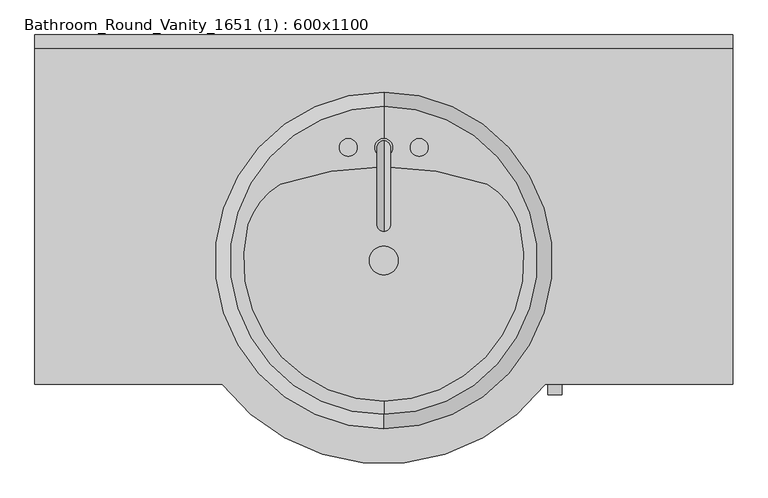
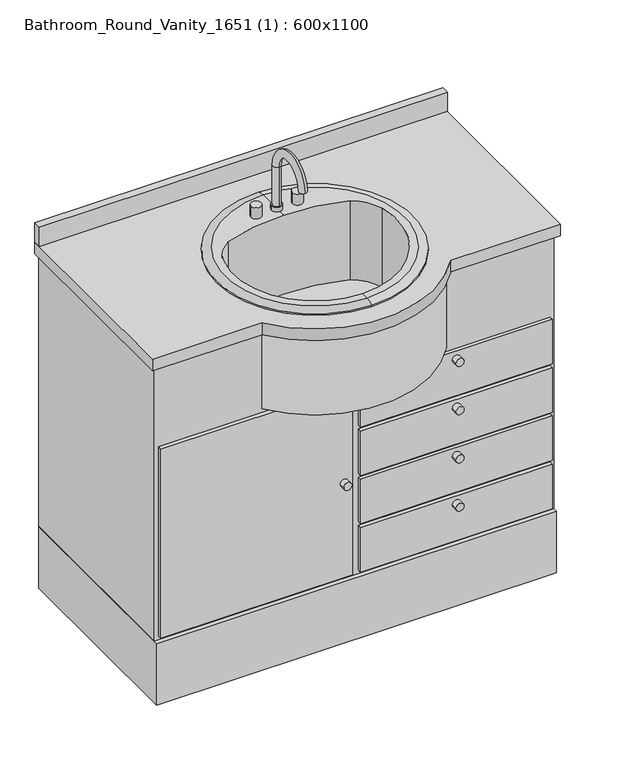
"""IFC4 building model written with IfcOpenShell, lengths in millimetres: furniture geometry, Bathroom_Round_Vanity_1651 (1) : 600x1100."""

import ifcopenshell
import ifcopenshell.guid

model = None  # the IFC model being written
_history = None  # IfcOwnerHistory: only IFC2X3 demands one
_inside = {}  # id of a spatial element -> (the spatial element, [elements in it])
_under = {}  # id of a project, library or spatial element -> (it, [spatial elements below it])
_declared = {}  # id of a project -> (the project, [libraries it declares])
_typed = {}  # id of a type object -> (the type object, [elements of that type])
_made_of = {}  # id of a material, layer set ... -> (it, [elements and type objects made of it])


def new_model(schema):
    """Start an empty IFC model of exactly this schema.

    Asked for "IFC4X3", IfcOpenShell would pick the latest addendum, in which some entities
    have other attributes; the version numbers below select the first issue.
    IFC2X3 requires an IfcOwnerHistory on every rooted entity: one is made here for all.
    """
    global model, _history
    if schema == "IFC4X3":
        model = ifcopenshell.file(schema_version=(4, 3, 0, 0))
    else:
        model = ifcopenshell.file(schema=schema)
    _inside.clear()
    _under.clear()
    _declared.clear()
    _typed.clear()
    _made_of.clear()
    _history = None
    if model.schema == "IFC2X3":
        org = make("IfcOrganization", Name="unknown")
        user = make(
            "IfcPersonAndOrganization",
            ThePerson=make("IfcPerson", FamilyName="unknown"),
            TheOrganization=org,
        )
        app = make(
            "IfcApplication",
            ApplicationDeveloper=org,
            Version="unknown",
            ApplicationFullName="unknown",
            ApplicationIdentifier="unknown",
        )
        _history = make(
            "IfcOwnerHistory",
            OwningUser=user,
            OwningApplication=app,
            ChangeAction="ADDED",
            CreationDate=0,
        )
    return model


def make(cls, **values):
    """One entity of the class cls with the attributes given. An attribute that is None is left unset."""
    return model.create_entity(
        cls, **{name: value for name, value in values.items() if value is not None}
    )


def rooted(cls, **values):
    """An entity with a GlobalId (a new one), such as an element, a storey or a relation."""
    return make(cls, GlobalId=ifcopenshell.guid.new(), OwnerHistory=_history, **values)


def si_unit(unit_type, name, prefix=None):
    """IfcSIUnit, for example si_unit("LENGTHUNIT", "METRE", prefix="MILLI")."""
    return make("IfcSIUnit", UnitType=unit_type, Prefix=prefix, Name=name)


def assignment(units):
    """IfcUnitAssignment: the units of a project."""
    return None if units is None else make("IfcUnitAssignment", Units=units)


def point(xyz):
    """IfcCartesianPoint."""
    return None if xyz is None else make("IfcCartesianPoint", Coordinates=xyz)


def direction(xyz):
    """IfcDirection."""
    return None if xyz is None else make("IfcDirection", DirectionRatios=xyz)


def frame(location, z_axis=None, x_axis=None):
    """IfcAxis2Placement3D, a coordinate frame: its origin and axes. An axis left out is left unset."""
    return make(
        "IfcAxis2Placement3D",
        Location=point(location),
        Axis=direction(z_axis),
        RefDirection=direction(x_axis),
    )


def frame_2d(location, x_axis=None):
    """IfcAxis2Placement2D, a coordinate frame in the plane: its origin and x axis."""
    return make(
        "IfcAxis2Placement2D", Location=point(location), RefDirection=direction(x_axis)
    )


def origin():
    """The frame at (0, 0, 0) with its axes left unset."""
    return frame((0.0, 0.0, 0.0))


def origin_with_axes():
    """The frame at (0, 0, 0) with the z axis (0, 0, 1) and the x axis (1, 0, 0) written out."""
    return frame((0.0, 0.0, 0.0), z_axis=(0.0, 0.0, 1.0), x_axis=(1.0, 0.0, 0.0))


def place(relative_to, where):
    """IfcLocalPlacement: puts the frame where relative to a parent placement (None: the world)."""
    return make(
        "IfcLocalPlacement", PlacementRelTo=relative_to, RelativePlacement=where
    )


def context(
    kind, dimensions, precision=None, world=None, true_north=None, identifier=None
):
    """IfcGeometricRepresentationContext, for example the 3D "Model" context."""
    return make(
        "IfcGeometricRepresentationContext",
        ContextIdentifier=identifier,
        ContextType=kind,
        CoordinateSpaceDimension=dimensions,
        Precision=precision,
        WorldCoordinateSystem=world,
        TrueNorth=true_north,
    )


def project(units=None, contexts=None):
    """IfcProject with its units and contexts."""
    return rooted(
        "IfcProject",
        Name="project",
        RepresentationContexts=contexts,
        UnitsInContext=assignment(units),
    )


def spatial(cls, under=None, at=None, **own):
    """A site, building, storey or space (cls), placed at a placement, below another one or the project."""
    s = rooted(cls, ObjectPlacement=at, **own)
    if under is not None:
        _under.setdefault(under.id(), (under, []))[1].append(s)
    return s


def polyline(points):
    """IfcPolyline through the points."""
    return make("IfcPolyline", Points=[point(p) for p in points])


def circle_curve(where, radius):
    """IfcCircle in the frame where."""
    return make("IfcCircle", Position=where, Radius=radius)


def ellipse_curve(where, semi_axis1, semi_axis2):
    """IfcEllipse in the frame where."""
    return make(
        "IfcEllipse", Position=where, SemiAxis1=semi_axis1, SemiAxis2=semi_axis2
    )


def trimmed(basis, trim1, trim2, sense, master):
    """IfcTrimmedCurve: the piece of a basis curve between two trims."""
    return make(
        "IfcTrimmedCurve",
        BasisCurve=basis,
        Trim1=trim1,
        Trim2=trim2,
        SenseAgreement=sense,
        MasterRepresentation=master,
    )


def segment(curve, same_sense, transition):
    """IfcCompositeCurveSegment."""
    return make(
        "IfcCompositeCurveSegment",
        Transition=transition,
        SameSense=same_sense,
        ParentCurve=curve,
    )


def composite_curve(segments, self_intersect=None):
    """IfcCompositeCurve: segments joined end to end."""
    return make("IfcCompositeCurve", Segments=segments, SelfIntersect=self_intersect)


def outline(outer, holes=None, kind="AREA"):
    """IfcArbitraryClosedProfileDef: a profile drawn as a closed curve; with holes, ...WithVoids."""
    if holes is None:
        return make("IfcArbitraryClosedProfileDef", ProfileType=kind, OuterCurve=outer)
    return make(
        "IfcArbitraryProfileDefWithVoids",
        ProfileType=kind,
        OuterCurve=outer,
        InnerCurves=holes,
    )


def extrude(swept, where, along, depth):
    """IfcExtrudedAreaSolid: the profile swept, set in the frame where, extruded along a direction by depth."""
    return make(
        "IfcExtrudedAreaSolid",
        SweptArea=swept,
        Position=where,
        ExtrudedDirection=direction(along),
        Depth=depth,
    )


def shape(context_of_items, identifier, shape_type, items):
    """IfcShapeRepresentation: the items that make up one representation, for example the "Body"."""
    return make(
        "IfcShapeRepresentation",
        ContextOfItems=context_of_items,
        RepresentationIdentifier=identifier,
        RepresentationType=shape_type,
        Items=items,
    )


def source(mapping_origin, context_of_items, identifier, shape_type, items):
    """IfcRepresentationMap: a shape defined once, which mapped items show again and again."""
    return make(
        "IfcRepresentationMap",
        MappingOrigin=mapping_origin,
        MappedRepresentation=shape(context_of_items, identifier, shape_type, items),
    )


def transform(
    local_origin,
    x_axis=None,
    y_axis=None,
    z_axis=None,
    scale=None,
    scale2=None,
    scale3=None,
    uniform=True,
):
    """IfcCartesianTransformationOperator3D, or its non-uniform kind. x_axis, y_axis, z_axis: its Axis1, 2, 3."""
    if uniform:
        return make(
            "IfcCartesianTransformationOperator3D",
            Axis1=direction(x_axis),
            Axis2=direction(y_axis),
            LocalOrigin=point(local_origin),
            Scale=scale,
            Axis3=direction(z_axis),
        )
    return make(
        "IfcCartesianTransformationOperator3DnonUniform",
        Axis1=direction(x_axis),
        Axis2=direction(y_axis),
        LocalOrigin=point(local_origin),
        Scale=scale,
        Axis3=direction(z_axis),
        Scale2=scale2,
        Scale3=scale3,
    )


def mapped(mapping_source, mapping_target):
    """IfcMappedItem: shows the shape of a source again, moved by a transform."""
    return make(
        "IfcMappedItem", MappingSource=mapping_source, MappingTarget=mapping_target
    )


def made_of(thing, what):
    """Note that an element or type object is made of a material, layer set ...; save() writes the relation."""
    if what is not None:
        _made_of.setdefault(what.id(), (what, []))[1].append(thing)
    return thing


def element(
    cls,
    number,
    at=None,
    inside=None,
    cuts=None,
    type_object=None,
    material=None,
    context=None,
    identifier="Body",
    shape_type=None,
    held_by="IfcProductDefinitionShape",
    body=None,
    shapes=None,
    **own,
):
    """One element of the class cls, such as IfcWall. Its Tag is "e" and its number.

    at: its placement. inside: the storey or other place that contains it. cuts: it is an
    opening in that element (IfcRelVoidsElement). A single representation is given by context,
    identifier, shape_type and body (its items); several are given by shapes. held_by: the class
    of the entity that holds the representations. save() writes the other relations.
    """
    e = rooted(cls, Tag="e%d" % number, ObjectPlacement=at, **own)
    if body is not None:
        shapes = [shape(context, identifier, shape_type, body)]
    if shapes is not None:
        e.Representation = make(held_by, Representations=shapes)
    if inside is not None:
        _inside.setdefault(inside.id(), (inside, []))[1].append(e)
    if cuts is not None:
        rooted(
            "IfcRelVoidsElement", RelatingBuildingElement=cuts, RelatedOpeningElement=e
        )
    if type_object is not None:
        _typed.setdefault(type_object.id(), (type_object, []))[1].append(e)
    return made_of(e, material)


def aggregate(whole, parts):
    """IfcRelAggregates: a whole, such as a stair, and the parts it consists of."""
    return rooted("IfcRelAggregates", RelatingObject=whole, RelatedObjects=parts)


def save(model, path):
    """Write the relations noted so far, then the file.

    IfcRelAggregates (storeys below a building ...), IfcRelContainedInSpatialStructure (elements
    in a storey), IfcRelDefinesByType, IfcRelAssociatesMaterial and IfcRelDeclares: one each for
    every whole, place, type object, material and project.
    """
    for whole, parts in _under.values():
        aggregate(whole, parts)
    for where, things in _inside.values():
        rooted(
            "IfcRelContainedInSpatialStructure",
            RelatedElements=things,
            RelatingStructure=where,
        )
    for kind, things in _typed.values():
        rooted("IfcRelDefinesByType", RelatedObjects=things, RelatingType=kind)
    for what, things in _made_of.values():
        rooted("IfcRelAssociatesMaterial", RelatedObjects=things, RelatingMaterial=what)
    for by, libraries in _declared.values():
        rooted("IfcRelDeclares", RelatingContext=by, RelatedDefinitions=libraries)
    model.write(path)


def plane_surface(at):
    """IfcPlane: the flat surface through the origin of the frame at, square to its z axis."""
    return make("IfcPlane", Position=at)


def cylinder_surface(at, radius):
    """IfcCylindricalSurface: all points at the distance radius from the z axis of the frame at."""
    return make("IfcCylindricalSurface", Position=at, Radius=radius)


def revolved_surface(curve, axis_point, axis_direction):
    """IfcSurfaceOfRevolution: the curve turned about the line through axis_point along axis_direction."""
    return make(
        "IfcSurfaceOfRevolution",
        SweptCurve=make("IfcArbitraryOpenProfileDef", ProfileType="CURVE", Curve=curve),
        AxisPosition=make("IfcAxis1Placement", Location=point(axis_point), Axis=direction(axis_direction)),
    )


def advanced_brep(points, edges, surfaces, faces):
    """IfcAdvancedBrep: a solid bounded by faces that lie on surfaces and meet in shared edges.

    An edge is (start, end): straight between two places in points (the first is 0);
    or (start, end, curve); or (start, end, curve, False) where it runs against its curve.
    A face is (place in surfaces, loops), or (place, loops, False) where it looks against
    its surface's normal. A loop lists edges by number (the first is 1), with a minus sign
    where the edge is run from its end to its start. The first loop is the outer one.
    """
    corners = [point(p) for p in points]
    vertices = [make("IfcVertexPoint", VertexGeometry=c) for c in corners]
    made = []
    for start, end, *more in edges:
        made.append(
            make(
                "IfcEdgeCurve",
                EdgeStart=vertices[start],
                EdgeEnd=vertices[end],
                EdgeGeometry=more[0] if more else make("IfcPolyline", Points=[corners[start], corners[end]]),
                SameSense=more[1] if len(more) > 1 else True,
            )
        )
    hull = []
    for where, loops, *sense in faces:
        bounds = []
        for j, loop in enumerate(loops):
            ring = [make("IfcOrientedEdge", EdgeElement=made[abs(k) - 1], Orientation=k > 0) for k in loop]
            bounds.append(
                make(
                    "IfcFaceOuterBound" if j == 0 else "IfcFaceBound",
                    Bound=make("IfcEdgeLoop", EdgeList=ring),
                    Orientation=True,
                )
            )
        hull.append(make("IfcAdvancedFace", Bounds=bounds, FaceSurface=surfaces[where], SameSense=sense[0] if sense else True))
    return make("IfcAdvancedBrep", Outer=make("IfcClosedShell", CfsFaces=hull))


def bathroom_round_vanity_1651_1_600x1100_b041f343(model_context):
    return source(origin(), model_context, "Body", "SolidModel", [
        advanced_brep(
        [(94.9377049, -170.6504315, 909.525), (94.9377049, -151.6004315, 909.525), (94.9377049, -170.6504315, 1022.2375), (94.9377049, -151.6004315, 1022.2375), (94.9377049, -262.4406462, 1022.2375), (94.9377049, -281.4906462, 1022.2375)],
        [
            (0, 1, circle_curve(frame((94.9377049, -161.1254315, 909.525), z_axis=(0.0, 0.0, -1.0), x_axis=(0.0, 1.0, 0.0)), 9.525)),
            (1, 0, circle_curve(frame((94.9377049, -161.1254315, 909.525), z_axis=(0.0, 0.0, -1.0), x_axis=(0.0, 1.0, 0.0)), 9.525)),
            (0, 2),
            (2, 3, circle_curve(frame((94.9377049, -161.1254315, 1022.2375), z_axis=(0.0, 0.0, -1.0), x_axis=(0.0, 1.0, 0.0)), 9.525)),
            (3, 1),
            (3, 2, circle_curve(frame((94.9377049, -161.1254315, 1022.2375), z_axis=(0.0, 0.0, -1.0), x_axis=(0.0, 1.0, 0.0)), 9.525)),
            (4, 5, circle_curve(frame((94.9377049, -271.9656462, 1022.2375), z_axis=(0.0, 0.0, -1.0), x_axis=(0.0, -1.0, 0.0)), 9.525)),
            (5, 4, circle_curve(frame((94.9377049, -271.9656462, 1022.2375), z_axis=(0.0, 0.0, -1.0), x_axis=(0.0, -1.0, 0.0)), 9.525)),
            (5, 3, circle_curve(frame((94.9377049, -216.5455388, 1022.2375), z_axis=(-1.0, 0.0, 0.0), x_axis=(0.0, 1.0, 0.0)), 64.9451073)),
            (2, 4, circle_curve(frame((94.9377049, -216.5455388, 1022.2375), z_axis=(1.0, 0.0, 0.0), x_axis=(0.0, 1.0, 0.0)), 45.8951073)),
        ],
        [
            plane_surface(frame((94.9377049, -170.6504315, 909.525), z_axis=(0.0, 0.0, -1.0), x_axis=(1.0, 0.0, 0.0))),
            cylinder_surface(frame((94.9377049, -161.1254315, 909.525), z_axis=(0.0, 0.0, -1.0), x_axis=(0.0, 1.0, 0.0)), 9.525),
            plane_surface(frame((94.9377049, -216.5455388, 1022.2375), z_axis=(0.0, 0.0, -1.0), x_axis=(0.0, -1.0, 0.0))),
            revolved_surface(trimmed(ellipse_curve(frame((94.9377049, -161.1254315, 1022.2375), z_axis=(0.0, 0.0, -1.0), x_axis=(0.0, 1.0, 0.0)), 9.525, 9.525), [point((94.9377049, -170.6504315, 1022.2375))], [point((94.9377049, -151.6004315, 1022.2375))], True, "CARTESIAN"), (94.9377049, -216.5455388, 1022.2375), (1.0, 0.0, 0.0)),
            revolved_surface(trimmed(ellipse_curve(frame((94.9377049, -161.1254315, 1022.2375), z_axis=(0.0, 0.0, -1.0), x_axis=(0.0, 1.0, 0.0)), 9.525, 9.525), [point((94.9377049, -151.6004315, 1022.2375))], [point((94.9377049, -170.6504315, 1022.2375))], True, "CARTESIAN"), (94.9377049, -216.5455388, 1022.2375), (1.0, 0.0, 0.0)),
        ],
        [
            (0, [[1, 2]]),
            (1, [[-1, 3, 4, 5]]),
            (1, [[-2, -5, 6, -3]]),
            (2, [[7, 8]]),
            (3, [[9, -4, 10, -8]]),
            (4, [[-10, -6, -9, -7]]),
        ],
    ),
        extrude(outline(composite_curve([segment(trimmed(circle_curve(frame_2d((94.9377049, -161.1254315)), 12.7), [point((82.2377049, -161.1254315))], [point((107.6377049, -161.1254315))], False, "CARTESIAN"), True, "CONTINUOUS"), segment(trimmed(circle_curve(frame_2d((94.9377049, -161.1254315)), 12.7), [point((107.6377049, -161.1254315))], [point((82.2377049, -161.1254315))], False, "CARTESIAN"), True, "CONTINUOUS")], self_intersect=False)), frame((0.0, 0.0, 909.525), z_axis=(0.0, 0.0, 1.0), x_axis=(1.0, 0.0, 0.0)), (0.0, 0.0, 1.0), 12.2352909),
        extrude(outline(composite_curve([segment(trimmed(circle_curve(frame_2d((44.1377049, -161.1254315)), 12.7), [point((31.4377049, -161.1254315))], [point((56.8377049, -161.1254315))], False, "CARTESIAN"), True, "CONTINUOUS"), segment(trimmed(circle_curve(frame_2d((44.1377049, -161.1254315)), 12.7), [point((56.8377049, -161.1254315))], [point((31.4377049, -161.1254315))], False, "CARTESIAN"), True, "CONTINUOUS")], self_intersect=False)), frame((0.0, 0.0, 909.525), z_axis=(0.0, 0.0, 1.0), x_axis=(1.0, 0.0, 0.0)), (0.0, 0.0, 1.0), 28.575),
        extrude(outline(composite_curve([segment(trimmed(circle_curve(frame_2d((145.7377049, -161.1254315)), 12.7), [point((133.0377049, -161.1254315))], [point((158.4377049, -161.1254315))], False, "CARTESIAN"), True, "CONTINUOUS"), segment(trimmed(circle_curve(frame_2d((145.7377049, -161.1254315)), 12.7), [point((158.4377049, -161.1254315))], [point((133.0377049, -161.1254315))], False, "CARTESIAN"), True, "CONTINUOUS")], self_intersect=False)), frame((0.0, 0.0, 909.525), z_axis=(0.0, 0.0, 1.0), x_axis=(1.0, 0.0, 0.0)), (0.0, 0.0, 1.0), 28.575),
        extrude(outline(composite_curve([segment(trimmed(circle_curve(frame_2d((94.9377049, -323.0504315)), 20.6375), [point((74.3002049, -323.0504315))], [point((115.5752049, -323.0504315))], False, "CARTESIAN"), True, "CONTINUOUS"), segment(trimmed(circle_curve(frame_2d((94.9377049, -323.0504315)), 20.6375), [point((115.5752049, -323.0504315))], [point((74.3002049, -323.0504315))], False, "CARTESIAN"), True, "CONTINUOUS")], self_intersect=False)), frame((0.0, 0.0, 684.1), z_axis=(0.0, 0.0, 1.0), x_axis=(1.0, 0.0, 0.0)), (0.0, 0.0, 1.0), 21.1842611),
        advanced_brep(
        [(94.9377049, -543.6051593, 909.525), (94.9377049, -102.4957037, 909.525), (94.9377049, -81.7504315, 903.96875), (94.9377049, -564.3504315, 903.96875), (94.9377049, -524.4587205, 909.525), (-99.884377, -271.9656462, 909.525), (-53.8675289, -214.1320102, 909.525), (94.9377049, -188.9519451, 909.525), (243.7429387, -214.1320102, 909.525), (289.7597868, -271.9656462, 909.525), (94.9377049, -515.3445528, 684.1), (94.9377049, -130.7563102, 684.1), (94.9377049, -323.0504315, 684.1), (94.9377049, -535.9008861, 705.2842611), (94.9377049, -110.1999769, 705.2842611), (94.9377049, -552.4441815, 900.0), (94.9377049, -93.6566815, 900.0), (94.9377049, -564.3504315, 900.0), (94.9377049, -81.7504315, 900.0), (243.7429387, -214.1320102, 705.2842611), (-53.8675289, -214.1320102, 705.2842611), (-99.884377, -271.9656462, 705.2842611), (289.7597868, -271.9656462, 705.2842611)],
        [
            (0, 1, circle_curve(frame((94.9377049, -323.0504315, 909.525), z_axis=(0.0, 0.0, -1.0), x_axis=(0.0, 1.0, 0.0)), 220.5547278)),
            (1, 2, circle_curve(frame((94.9377049, -98.7806884, 881.889434), z_axis=(-1.0, 0.0, 0.0), x_axis=(0.0, 1.0, 0.0)), 27.8841505)),
            (2, 3, circle_curve(frame((94.9377049, -323.0504315, 903.96875), z_axis=(0.0, 0.0, 1.0), x_axis=(0.0, 1.0, 0.0)), 241.3)),
            (3, 0, circle_curve(frame((94.9377049, -547.3201745, 881.889434), z_axis=(-1.0, 0.0, 0.0), x_axis=(0.0, -1.0, 0.0)), 27.8841505)),
            (1, 0, circle_curve(frame((94.9377049, -323.0504315, 909.525), z_axis=(0.0, 0.0, -1.0), x_axis=(0.0, 1.0, 0.0)), 220.5547278)),
            (3, 2, circle_curve(frame((94.9377049, -323.0504315, 903.96875), z_axis=(0.0, 0.0, 1.0), x_axis=(0.0, 1.0, 0.0)), 241.3)),
            (0, 4),
            (4, 5, circle_curve(frame((94.9377049, -323.0504315, 909.525), z_axis=(0.0, 0.0, -1.0), x_axis=(1.0, 0.0, 0.0)), 201.408289)),
            (5, 6, circle_curve(frame((-0.3450667, -303.9426335, 909.525), z_axis=(0.0, 0.0, -1.0), x_axis=(1.0, 0.0, 0.0)), 104.5495194)),
            (6, 7, circle_curve(frame((94.9377049, -641.2349961, 909.525), z_axis=(0.0, 0.0, -1.0), x_axis=(1.0, 0.0, 0.0)), 452.283051)),
            (7, 1),
            (7, 8, circle_curve(frame((94.9377049, -641.2349961, 909.525), z_axis=(0.0, 0.0, -1.0), x_axis=(1.0, 0.0, 0.0)), 452.283051)),
            (8, 9, circle_curve(frame((190.2204765, -303.9426335, 909.525), z_axis=(0.0, 0.0, -1.0), x_axis=(1.0, 0.0, 0.0)), 104.5495194)),
            (9, 4, circle_curve(frame((94.9377049, -323.0504315, 909.525), z_axis=(0.0, 0.0, -1.0), x_axis=(1.0, 0.0, 0.0)), 201.408289)),
            (10, 11, circle_curve(frame((94.9377049, -323.0504315, 684.1), z_axis=(0.0, 0.0, -1.0), x_axis=(0.0, 1.0, 0.0)), 192.2941213)),
            (11, 12),
            (12, 10),
            (11, 10, circle_curve(frame((94.9377049, -323.0504315, 684.1), z_axis=(0.0, 0.0, -1.0), x_axis=(0.0, 1.0, 0.0)), 192.2941213)),
            (10, 13, circle_curve(frame((94.9377049, -515.3445528, 704.6656396), z_axis=(-1.0, 0.0, 0.0), x_axis=(0.0, -1.0, 0.0)), 20.5656396)),
            (13, 14, circle_curve(frame((94.9377049, -323.0504315, 705.2842611), z_axis=(0.0, 0.0, -1.0), x_axis=(0.0, 1.0, 0.0)), 212.8504546)),
            (14, 11, circle_curve(frame((94.9377049, -130.7563102, 704.6656396), z_axis=(-1.0, 0.0, 0.0), x_axis=(0.0, 1.0, 0.0)), 20.5656396)),
            (14, 13, circle_curve(frame((94.9377049, -323.0504315, 705.2842611), z_axis=(0.0, 0.0, -1.0), x_axis=(0.0, 1.0, 0.0)), 212.8504546)),
            (13, 15),
            (15, 16, circle_curve(frame((94.9377049, -323.0504315, 900.0), z_axis=(0.0, 0.0, -1.0), x_axis=(0.0, 1.0, 0.0)), 229.39375)),
            (16, 14),
            (16, 15, circle_curve(frame((94.9377049, -323.0504315, 900.0), z_axis=(0.0, 0.0, -1.0), x_axis=(0.0, 1.0, 0.0)), 229.39375)),
            (15, 17),
            (17, 18, circle_curve(frame((94.9377049, -323.0504315, 900.0), z_axis=(0.0, 0.0, -1.0), x_axis=(0.0, 1.0, 0.0)), 241.3)),
            (18, 16),
            (18, 17, circle_curve(frame((94.9377049, -323.0504315, 900.0), z_axis=(0.0, 0.0, -1.0), x_axis=(0.0, 1.0, 0.0)), 241.3)),
            (2, 18),
            (17, 3),
            (19, 20, circle_curve(frame((94.9377049, -641.2349961, 705.2842611), z_axis=(0.0, 0.0, 1.0), x_axis=(1.0, 0.0, 0.0)), 452.283051)),
            (20, 21, circle_curve(frame((-0.3450667, -303.9426335, 705.2842611), z_axis=(0.0, 0.0, 1.0), x_axis=(1.0, 0.0, 0.0)), 104.5495194)),
            (21, 22, circle_curve(frame((94.9377049, -323.0504315, 705.2842611), z_axis=(0.0, 0.0, 1.0), x_axis=(1.0, 0.0, 0.0)), 201.408289)),
            (22, 19, circle_curve(frame((190.2204765, -303.9426335, 705.2842611), z_axis=(0.0, 0.0, 1.0), x_axis=(1.0, 0.0, 0.0)), 104.5495194)),
            (19, 8),
            (6, 20),
            (5, 21),
            (9, 22),
        ],
        [
            revolved_surface(trimmed(ellipse_curve(frame((94.9377049, -98.7806884, 881.889434), z_axis=(1.0, 0.0, 0.0), x_axis=(0.0, 1.0, 0.0)), 27.8841505, 27.8841505), [point((94.9377049, -81.7504315, 903.96875))], [point((94.9377049, -102.4957037, 909.525))], True, "CARTESIAN"), (94.9377049, -323.0504315, 909.525), (0.0, 0.0, 1.0)),
            plane_surface(frame((94.9377049, -323.0504315, 909.525), z_axis=(0.0, 0.0, 1.0), x_axis=(0.0, 1.0, 0.0))),
            plane_surface(frame((94.9377049, -323.0504315, 684.1), z_axis=(0.0, 0.0, -1.0), x_axis=(0.0, 1.0, 0.0))),
            revolved_surface(trimmed(ellipse_curve(frame((94.9377049, -130.7563102, 704.6656396), z_axis=(1.0, 0.0, 0.0), x_axis=(0.0, 1.0, 0.0)), 20.5656396, 20.5656396), [point((94.9377049, -130.7563102, 684.1))], [point((94.9377049, -110.1999769, 705.2842611))], True, "CARTESIAN"), (94.9377049, -323.0504315, 909.525), (0.0, 0.0, 1.0)),
            revolved_surface(polyline([(94.9377049, -110.1999769, 705.2842611), (94.9377049, -93.6566815, 900.0)]), (94.9377049, -323.0504315, 909.525), (0.0, 0.0, 1.0)),
            plane_surface(frame((94.9377049, -323.0504315, 900.0), z_axis=(0.0, 0.0, -1.0), x_axis=(0.0, 1.0, 0.0))),
            cylinder_surface(frame((94.9377049, -323.0504315, 909.525), z_axis=(0.0, 0.0, 1.0), x_axis=(0.0, 1.0, 0.0)), 241.3),
            plane_surface(frame((547.2207559, -641.2349961, 705.2842611), z_axis=(0.0, 0.0, 1.0), x_axis=(0.0, -1.0, 0.0))),
            revolved_surface(polyline([(547.2207559, -641.2349961, 909.525), (547.2207559, -641.2349961, 705.2842611)]), (94.9377049, -641.2349961, 705.2842611), (0.0, 0.0, 1.0)),
            revolved_surface(polyline([(104.20445269999999, -303.9426335, 909.525), (104.20445269999999, -303.9426335, 705.2842611)]), (-0.3450667, -303.9426335, 705.2842611), (0.0, 0.0, 1.0)),
            revolved_surface(polyline([(296.3459939, -323.0504315, 909.525), (296.3459939, -323.0504315, 705.2842611)]), (94.9377049, -323.0504315, 705.2842611), (0.0, 0.0, 1.0)),
            revolved_surface(polyline([(294.76999589999997, -303.9426335, 909.525), (294.76999589999997, -303.9426335, 705.2842611)]), (190.2204765, -303.9426335, 705.2842611), (0.0, 0.0, 1.0)),
        ],
        [
            (0, [[1, 2, 3, 4]]),
            (0, [[-2, 5, -4, 6]]),
            (1, [[-1, 7, 8, 9, 10, 11]]),
            (1, [[-5, -11, 12, 13, 14, -7]]),
            (2, [[15, 16, 17]]),
            (2, [[-16, 18, -17]]),
            (3, [[-15, 19, 20, 21]]),
            (3, [[-18, -21, 22, -19]]),
            (4, [[-20, 23, 24, 25]]),
            (4, [[-22, -25, 26, -23]]),
            (5, [[-24, 27, 28, 29]]),
            (5, [[-26, -29, 30, -27]]),
            (6, [[-3, 31, -28, 32]]),
            (6, [[-6, -32, -30, -31]]),
            (7, [[33, 34, 35, 36]]),
            (8, [[-33, 37, -12, -10, 38]]),
            (9, [[-34, -38, -9, 39]]),
            (10, [[-35, -39, -8, -14, 40]]),
            (11, [[-36, -40, -13, -37]]),
        ],
    ),
        extrude(outline(composite_curve([segment(trimmed(circle_curve(frame_2d((640.0, 339.9377049)), 10.0), [point((640.0, 329.9377049))], [point((640.0, 349.9377049))], False, "CARTESIAN"), True, "CONTINUOUS"), segment(trimmed(circle_curve(frame_2d((640.0, 339.9377049)), 10.0), [point((640.0, 349.9377049))], [point((640.0, 329.9377049))], False, "CARTESIAN"), True, "CONTINUOUS")], self_intersect=False)), frame((0.0, -515.0, 0.0), z_axis=(0.0, 1.0, 0.0), x_axis=(0.0, 0.0, 1.0)), (0.0, 0.0, 1.0), 15.0),
        extrude(outline(composite_curve([segment(trimmed(circle_curve(frame_2d((515.0, 339.9377049)), 10.0), [point((515.0, 329.9377049))], [point((515.0, 349.9377049))], False, "CARTESIAN"), True, "CONTINUOUS"), segment(trimmed(circle_curve(frame_2d((515.0, 339.9377049)), 10.0), [point((515.0, 349.9377049))], [point((515.0, 329.9377049))], False, "CARTESIAN"), True, "CONTINUOUS")], self_intersect=False)), frame((0.0, -515.0, 0.0), z_axis=(0.0, 1.0, 0.0), x_axis=(0.0, 0.0, 1.0)), (0.0, 0.0, 1.0), 15.0),
        extrude(outline(composite_curve([segment(trimmed(circle_curve(frame_2d((390.0, 339.9377049)), 10.0), [point((390.0, 329.9377049))], [point((390.0, 349.9377049))], False, "CARTESIAN"), True, "CONTINUOUS"), segment(trimmed(circle_curve(frame_2d((390.0, 339.9377049)), 10.0), [point((390.0, 349.9377049))], [point((390.0, 329.9377049))], False, "CARTESIAN"), True, "CONTINUOUS")], self_intersect=False)), frame((0.0, -515.0, 0.0), z_axis=(0.0, 1.0, 0.0), x_axis=(0.0, 0.0, 1.0)), (0.0, 0.0, 1.0), 15.0),
        extrude(outline(composite_curve([segment(polyline([(594.9377049, 0.0), (594.9377049, -500.0), (326.334637, -500.0)]), True, "CONTINUOUS"), segment(trimmed(circle_curve(frame_2d((94.9377049, -323.0504315)), 291.3), [point((326.334637, -500.0))], [point((-136.4592272, -500.0))], False, "CARTESIAN"), True, "CONTINUOUS"), segment(polyline([(-136.4592272, -500.0), (-405.0622951, -500.0), (-405.0622951, 0.0), (594.9377049, 0.0)]), True, "CONTINUOUS")], self_intersect=False), holes=[composite_curve([segment(trimmed(circle_curve(frame_2d((94.9377049, -323.0504315)), 220.5547278), [point((94.9377049, -102.4957037))], [point((94.9377049, -543.6051593))], True, "CARTESIAN"), True, "CONTINUOUS"), segment(trimmed(circle_curve(frame_2d((94.9377049, -323.0504315)), 220.5547278), [point((94.9377049, -543.6051593))], [point((94.9377049, -102.4957037))], True, "CARTESIAN"), True, "CONTINUOUS")], self_intersect=False)]), frame((0.0, 0.0, 870.0), z_axis=(0.0, 0.0, 1.0), x_axis=(1.0, 0.0, 0.0)), (0.0, 0.0, 1.0), 30.0),
        extrude(outline(composite_curve([segment(trimmed(circle_curve(frame_2d((265.0, 339.9377049)), 10.0), [point((265.0, 329.9377049))], [point((265.0, 349.9377049))], False, "CARTESIAN"), True, "CONTINUOUS"), segment(trimmed(circle_curve(frame_2d((265.0, 339.9377049)), 10.0), [point((265.0, 349.9377049))], [point((265.0, 329.9377049))], False, "CARTESIAN"), True, "CONTINUOUS")], self_intersect=False)), frame((0.0, -515.0, 0.0), z_axis=(0.0, 1.0, 0.0), x_axis=(0.0, 0.0, 1.0)), (0.0, 0.0, 1.0), 15.0),
        extrude(outline(composite_curve([segment(trimmed(circle_curve(frame_2d((415.0, 64.9377049)), 10.0), [point((415.0, 74.9377049))], [point((415.0, 54.9377049))], False, "CARTESIAN"), True, "CONTINUOUS"), segment(trimmed(circle_curve(frame_2d((415.0, 64.9377049)), 10.0), [point((415.0, 54.9377049))], [point((415.0, 74.9377049))], False, "CARTESIAN"), True, "CONTINUOUS")], self_intersect=False)), frame((0.0, -515.0, 0.0), z_axis=(0.0, 1.0, 0.0), x_axis=(0.0, 0.0, 1.0)), (0.0, 0.0, 1.0), 15.0),
        extrude(outline(polyline([(574.9377049, -500.0), (104.9377049, -500.0), (104.9377049, -490.0), (574.9377049, -490.0), (574.9377049, -500.0)])), frame((0.0, 0.0, 170.0), z_axis=(0.0, 0.0, 1.0), x_axis=(1.0, 0.0, 0.0)), (0.0, 0.0, 1.0), 115.0),
        extrude(outline(polyline([(84.9377049, -500.0), (-385.0622951, -500.0), (-385.0622951, -490.0), (84.9377049, -490.0), (84.9377049, -500.0)])), frame((0.0, 0.0, 170.0), z_axis=(0.0, 0.0, 1.0), x_axis=(1.0, 0.0, 0.0)), (0.0, 0.0, 1.0), 490.0),
        extrude(outline(polyline([(574.9377049, -500.0), (104.9377049, -500.0), (104.9377049, -490.0), (574.9377049, -490.0), (574.9377049, -500.0)])), frame((0.0, 0.0, 545.0), z_axis=(0.0, 0.0, 1.0), x_axis=(1.0, 0.0, 0.0)), (0.0, 0.0, 1.0), 115.0),
        extrude(outline(polyline([(574.9377049, -500.0), (104.9377049, -500.0), (104.9377049, -490.0), (574.9377049, -490.0), (574.9377049, -500.0)])), frame((0.0, 0.0, 420.0), z_axis=(0.0, 0.0, 1.0), x_axis=(1.0, 0.0, 0.0)), (0.0, 0.0, 1.0), 115.0),
        extrude(outline(polyline([(574.9377049, -500.0), (104.9377049, -500.0), (104.9377049, -490.0), (574.9377049, -490.0), (574.9377049, -500.0)])), frame((0.0, 0.0, 295.0), z_axis=(0.0, 0.0, 1.0), x_axis=(1.0, 0.0, 0.0)), (0.0, 0.0, 1.0), 115.0),
        extrude(outline(polyline([(584.9377049, 0.0), (584.9377049, -500.0), (-395.0622951, -500.0), (-395.0622951, 0.0), (584.9377049, 0.0)])), origin_with_axes(), (0.0, 0.0, 1.0), 160.0),
        advanced_brep(
        [(321.3389672, -490.0, 670.0), (-131.4635574, -490.0, 670.0), (321.3389672, -490.0, 870.0), (584.9377049, -490.0, 870.0), (584.9377049, 0.0, 870.0), (-395.0622951, 0.0, 870.0), (-395.0622951, -490.0, 870.0), (-131.4635574, -490.0, 870.0), (316.2305492, -480.0, 870.0), (-126.3551394, -480.0, 870.0), (-385.0622951, -480.0, 870.0), (-385.0622951, -10.0, 870.0), (574.9377049, -10.0, 870.0), (574.9377049, -480.0, 870.0), (-395.0622951, -490.0, 160.0), (584.9377049, -490.0, 160.0), (-395.0622951, 0.0, 160.0), (584.9377049, 0.0, 160.0), (-126.3551394, -480.0, 680.0), (316.2305492, -480.0, 680.0), (574.9377049, -480.0, 160.0), (-385.0622951, -480.0, 160.0), (574.9377049, -10.0, 160.0), (-385.0622951, -10.0, 160.0)],
        [
            (0, 1, circle_curve(frame((94.9377049, -323.0504315, 670.0), z_axis=(0.0, 0.0, -1.0), x_axis=(0.0, -1.0, 0.0)), 281.3)),
            (1, 0),
            (2, 3),
            (3, 4),
            (4, 5),
            (5, 6),
            (6, 7),
            (7, 2, circle_curve(frame((94.9377049, -323.0504315, 870.0), z_axis=(0.0, 0.0, 1.0), x_axis=(0.0, -1.0, 0.0)), 281.3)),
            (8, 9, circle_curve(frame((94.9377049, -323.0504315, 870.0), z_axis=(0.0, 0.0, -1.0), x_axis=(0.0, -1.0, 0.0)), 271.3)),
            (9, 10),
            (10, 11),
            (11, 12),
            (12, 13),
            (13, 8),
            (0, 2),
            (7, 1),
            (6, 14),
            (14, 15),
            (15, 3),
            (5, 16),
            (16, 14),
            (4, 17),
            (17, 16),
            (15, 17),
            (9, 18),
            (18, 19),
            (19, 8),
            (13, 20),
            (20, 21),
            (21, 10),
            (12, 22),
            (22, 20),
            (11, 23),
            (23, 22),
            (21, 23),
            (19, 18, circle_curve(frame((94.9377049, -323.0504315, 680.0), z_axis=(0.0, 0.0, -1.0), x_axis=(0.0, -1.0, 0.0)), 271.3)),
        ],
        [
            plane_surface(frame((94.9377049, -604.3504315, 670.0), z_axis=(0.0, 0.0, -1.0), x_axis=(-1.0, 0.0, 0.0))),
            plane_surface(frame((94.9377049, -604.3504315, 870.0), z_axis=(0.0, 0.0, 1.0), x_axis=(1.0, 0.0, 0.0))),
            cylinder_surface(frame((94.9377049, -323.0504315, 870.0), z_axis=(0.0, 0.0, -1.0), x_axis=(0.0, -1.0, 0.0)), 281.3),
            plane_surface(frame((-131.4635574, -490.0, 670.0), z_axis=(0.0, -1.0, 0.0), x_axis=(0.0, 0.0, 1.0))),
            plane_surface(frame((-395.0622951, -490.0, 670.0), z_axis=(-1.0, 0.0, 0.0), x_axis=(0.0, 0.0, 1.0))),
            plane_surface(frame((-395.0622951, 0.0, 670.0), z_axis=(0.0, 1.0, 0.0), x_axis=(0.0, 0.0, 1.0))),
            plane_surface(frame((584.9377049, 0.0, 670.0), z_axis=(1.0, 0.0, 0.0), x_axis=(0.0, 0.0, 1.0))),
            plane_surface(frame((316.2305492, -480.0, 670.0), z_axis=(0.0, 1.0, 0.0), x_axis=(0.0, 0.0, 1.0))),
            plane_surface(frame((574.9377049, -480.0, 670.0), z_axis=(-1.0, 0.0, 0.0), x_axis=(0.0, 0.0, 1.0))),
            plane_surface(frame((574.9377049, -10.0, 670.0), z_axis=(0.0, -1.0, 0.0), x_axis=(0.0, 0.0, 1.0))),
            plane_surface(frame((-385.0622951, -10.0, 670.0), z_axis=(1.0, 0.0, 0.0), x_axis=(0.0, 0.0, 1.0))),
            revolved_surface(polyline([(94.9377049, -594.3504315, 870.0), (94.9377049, -594.3504315, 680.0)]), (94.9377049, -323.0504315, 870.0), (0.0, 0.0, 1.0)),
            plane_surface(frame((366.2377049, -323.0504315, 680.0), z_axis=(0.0, 0.0, 1.0), x_axis=(0.0, 1.0, 0.0))),
            plane_surface(frame((-395.0622951, 0.0, 160.0), z_axis=(0.0, 0.0, -1.0), x_axis=(1.0, 0.0, 0.0))),
        ],
        [
            (0, [[1, 2]]),
            (1, [[3, 4, 5, 6, 7, 8], [9, 10, 11, 12, 13, 14]]),
            (2, [[-1, 15, -8, 16]]),
            (3, [[-7, 17, 18, 19, -3, -15, -2, -16]]),
            (4, [[-17, -6, 20, 21]]),
            (5, [[-20, -5, 22, 23]]),
            (6, [[-22, -4, -19, 24]]),
            (7, [[-10, 25, 26, 27, -14, 28, 29, 30]]),
            (8, [[-28, -13, 31, 32]]),
            (9, [[-31, -12, 33, 34]]),
            (10, [[-33, -11, -30, 35]]),
            (11, [[-9, -27, 36, -25]]),
            (12, [[-26, -36]]),
            (13, [[-23, -24, -18, -21], [-35, -29, -32, -34]]),
        ],
    ),
        extrude(outline(polyline([(-405.0622951, -19.05), (-405.0622951, 0.0), (594.9377049, 0.0), (594.9377049, -19.05), (-405.0622951, -19.05)])), frame((0.0, 0.0, 900.0), z_axis=(0.0, 0.0, 1.0), x_axis=(1.0, 0.0, 0.0)), (0.0, 0.0, 1.0), 50.0),
    ])


if __name__ == "__main__":
    model = new_model("IFC4")
    model_context = context("Model", 3, world=origin())
    ifc_project = project(units=[si_unit("LENGTHUNIT", "METRE", prefix="MILLI")], contexts=[model_context])
    site = spatial("IfcSite", under=ifc_project)
    building = spatial("IfcBuilding", under=site)
    placement = place(None, origin())
    bathroom_round_vanity_1651_1_600x1100_shape = bathroom_round_vanity_1651_1_600x1100_b041f343(model_context)
    element("IfcFurniture", 1, ObjectType="Bathroom_Round_Vanity_1651 (1) : 600x1100", at=placement, inside=building, context=model_context, shape_type="MappedRepresentation", body=[
        mapped(bathroom_round_vanity_1651_1_600x1100_shape, transform((0.0, 0.0, 0.0), x_axis=(1.0, 0.0, 0.0), y_axis=(0.0, 1.0, 0.0), z_axis=(0.0, 0.0, 1.0))),
    ])
    save(model, "model.ifc")

# Revit data of these elements
# Type "Bathroom_Round_Vanity_1651 (1) : 600x1100"
#   Depth = 1' - 7.68504"
#   Height = 2' - 11.43307"
#   Plinth Depth = 0' - 1.37795"
#   Plinth Height = 0' - 6.29921"
#   Width = 3' - 3.37008"
#   Cabinet Material = Vanity-Body
#   Door/Drawer Material = Vanity-Body
#   Handle Material = Vanity-Push
#   Default Elevation = 0
# Element 1 (IfcFurniture, "Bathroom_Round_Vanity_1651 (1) : 600x1100")
#   Materials on its faces: "Vanity-Doors", "Vanity-Push", "Sink-Body", "Sink-Faucet", "Vanity-Top", "Vanity-Body"
# Materials
#   "Vanity-Body": class "Unassigned", colour RGB 255 255 255, transparency 0, Comments = "Rendering appearance not upgraded "
#   "Vanity-Push": class "Unassigned", colour RGB 0 0 0, transparency 0, Comments = "Rendering appearance not upgraded "
#   "Vanity-Doors": class "Unassigned", colour RGB 220 220 220, transparency 0, Comments = "Rendering appearance not upgraded "
#   "Sink-Body": class "Unassigned", colour RGB 250 244 225, transparency 0, Comments = "Rendering appearance not upgraded "
#   "Sink-Faucet": class "Unassigned", colour RGB 247 247 247, transparency 0, Comments = "Rendering appearance not upgraded "
#   "Vanity-Top": class "Unassigned", colour RGB 163 163 163, transparency 0, Comments = "Rendering appearance not upgraded "
